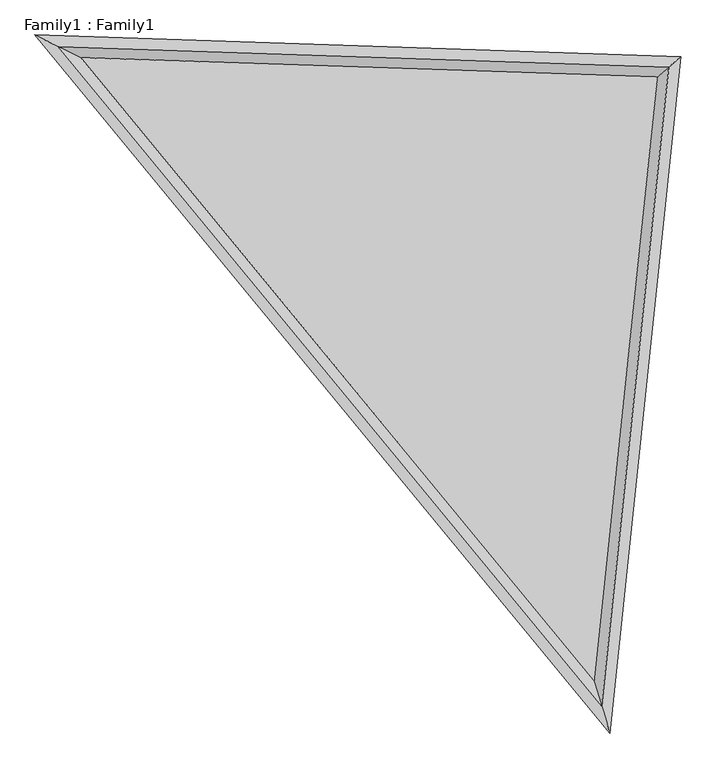
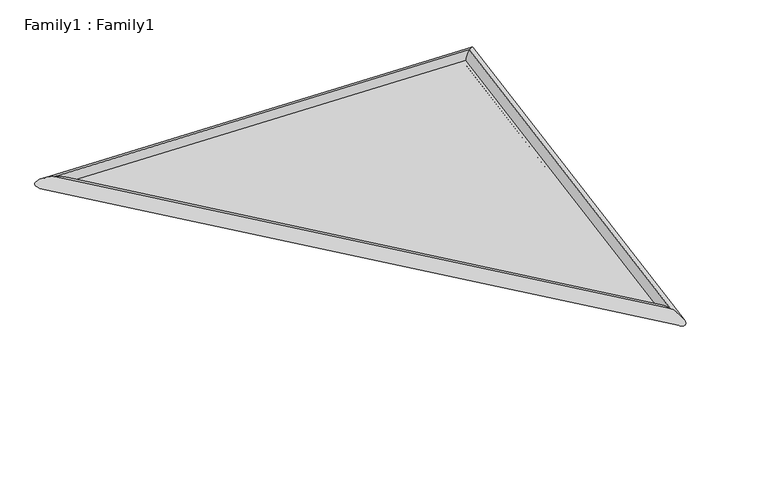
"""IFC4 building model written with IfcOpenShell, lengths in millimetres: proxy geometry, Family1 : Family1."""

from ifc_helpers import new_model, si_unit, frame, origin, origin_with_axes, place, context, project, spatial, polyline, ellipse_curve, outline, extrude, source, transform, mapped, element, save
from ifc_brep_helpers import cylinder_surface, advanced_brep


def family1_family1_f93d771a(model_context):
    return source(origin(), model_context, "Body", "SolidModel", [
        extrude(outline(polyline([(2391.8309811, -3543.2509634), (-2637.6447401, 2558.4492268), (3012.73621, 2368.7429415), (2391.8309811, -3543.2509634)])), origin_with_axes(), (0.0, 0.0, 1.0), 34.1328789),
        advanced_brep(
        [(2391.8309811, -3543.2509634, 100.0), (2391.8309811, -3543.2509634, -100.0), (-2637.6447401, 2558.4492268, -100.0), (-2637.6447401, 2558.4492268, 100.0), (3012.73621, 2368.7429415, -100.0), (3012.73621, 2368.7429415, 100.0)],
        [
            (0, 1, ellipse_curve(frame((2391.8309811, -3543.2509634, 0.0), z_axis=(-0.9575653329500438, -0.28821629574379004, 0.0), x_axis=(0.28821629574379, -0.9575653329500439, 0.0)), 258.6267019, 100.0)),
            (1, 2),
            (2, 3, ellipse_curve(frame((-2637.6447401, 2558.4492268, 0.0), z_axis=(-0.44170192490219773, -0.8971618636219963, 0.0), x_axis=(0.8971618636219962, -0.4417019249021976, 0.0)), 243.1027052, 100.0)),
            (3, 0),
            (1, 0, ellipse_curve(frame((2391.8309811, -3543.2509634, 0.0), z_axis=(-0.9575653329500438, -0.28821629574379004, 0.0), x_axis=(0.28821629574379, -0.9575653329500439, 0.0)), 258.6267019, 100.0)),
            (3, 2, ellipse_curve(frame((-2637.6447401, 2558.4492268, 0.0), z_axis=(-0.44170192490219773, -0.8971618636219963, 0.0), x_axis=(0.8971618636219962, -0.4417019249021976, 0.0)), 243.1027052, 100.0)),
            (2, 4),
            (4, 5, ellipse_curve(frame((3012.73621, 2368.7429415, 0.0), z_axis=(-0.656596146057357, 0.7542423357135463, 0.0), x_axis=(-0.7542423357135462, -0.6565961460573569, 0.0)), 146.7275817, 100.0)),
            (5, 3),
            (5, 4, ellipse_curve(frame((3012.73621, 2368.7429415, 0.0), z_axis=(-0.656596146057357, 0.7542423357135463, 0.0), x_axis=(-0.7542423357135462, -0.6565961460573569, 0.0)), 146.7275817, 100.0)),
            (4, 1),
            (0, 5),
        ],
        [
            cylinder_surface(frame((2391.8309811, -3543.2509634, 0.0), z_axis=(0.6360497753950819, -0.7716480306589696, 0.0), x_axis=(-0.7716480306589696, -0.6360497753950819, 0.0)), 100.0),
            cylinder_surface(frame((-2637.6447401, 2558.4492268, 0.0), z_axis=(-0.9994368669489655, 0.03355516328727677, 0.0), x_axis=(0.03355516328727677, 0.9994368669489655, 0.0)), 100.0),
            cylinder_surface(frame((3012.73621, 2368.7429415, 0.0), z_axis=(0.10445020082294756, 0.9945301179693081, 0.0), x_axis=(0.9945301179693081, -0.10445020082294756, 0.0)), 100.0),
        ],
        [
            (0, [[1, 2, 3, 4]]),
            (0, [[5, -4, 6, -2]]),
            (1, [[-3, 7, 8, 9]]),
            (1, [[-6, -9, 10, -7]]),
            (2, [[-8, 11, -1, 12]]),
            (2, [[-10, -12, -5, -11]]),
        ],
    ),
    ])


if __name__ == "__main__":
    model = new_model("IFC4")
    model_context = context("Model", 3, world=origin())
    ifc_project = project(units=[si_unit("LENGTHUNIT", "METRE", prefix="MILLI")], contexts=[model_context])
    site = spatial("IfcSite", under=ifc_project)
    building = spatial("IfcBuilding", under=site)
    placement = place(None, origin())
    family1_family1_shape = family1_family1_f93d771a(model_context)
    element("IfcBuildingElementProxy", 1, Name="Family1 : Family1", ObjectType="Family1 : Family1", at=placement, inside=building, context=model_context, shape_type="MappedRepresentation", body=[
        mapped(family1_family1_shape, transform((0.0, 0.0, 0.0), x_axis=(1.0, 0.0, 0.0), y_axis=(0.0, 1.0, 0.0), z_axis=(0.0, 0.0, 1.0))),
    ])
    save(model, "model.ifc")

# Revit data of these elements
# Type "Family1 : Family1"
#   Default Elevation = 0
# Element 1 (IfcBuildingElementProxy, "Family1 : Family1")
#   Materials on its faces: "Glass"
# Materials
#   "Glass": class "Glass", colour RGB 0 128 192, transparency 0.9, Description = "Soda Lime Glass", Cost = 0
